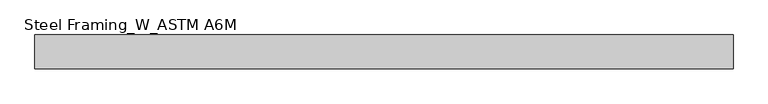
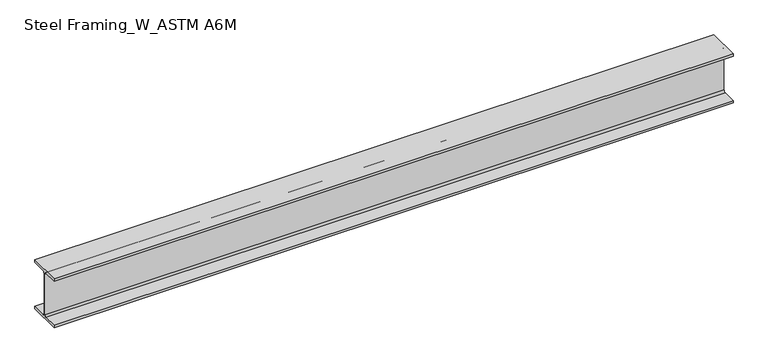
"""IFC4 building model written with IfcOpenShell, lengths in millimetres: beam geometry, Steel Framing_W_ASTM A6M : H_SB_AR_S02_W200x31.3_B6."""

from ifc_helpers import new_model, si_unit, point, frame, frame_2d, origin, place, context, project, spatial, polyline, circle_curve, trimmed, segment, composite_curve, outline, extrude, source, transform, mapped, element, save


def steel_framing_w_astm_a6m_88cf460a(model_context):
    return source(origin(), model_context, "Body", "SweptSolid", [
        extrude(outline(composite_curve([segment(polyline([(67.0, -94.8), (67.0, -105.0), (-67.0, -105.0), (-67.0, -94.8), (-10.775, -94.8)]), True, "CONTINUOUS"), segment(trimmed(circle_curve(frame_2d((-10.775, -87.2)), 7.6), [point((-10.775, -94.8))], [point((-3.175, -87.2))], True, "CARTESIAN"), True, "CONTINUOUS"), segment(polyline([(-3.175, -87.2), (-3.175, 87.2)]), True, "CONTINUOUS"), segment(trimmed(circle_curve(frame_2d((-10.775, 87.2)), 7.6), [point((-3.175, 87.2))], [point((-10.775, 94.8))], True, "CARTESIAN"), True, "CONTINUOUS"), segment(polyline([(-10.775, 94.8), (-67.0, 94.8), (-67.0, 105.0), (67.0, 105.0), (67.0, 94.8), (10.775, 94.8)]), True, "CONTINUOUS"), segment(trimmed(circle_curve(frame_2d((10.775, 87.2)), 7.6), [point((10.775, 94.8))], [point((3.175, 87.2))], True, "CARTESIAN"), True, "CONTINUOUS"), segment(polyline([(3.175, 87.2), (3.175, -87.2)]), True, "CONTINUOUS"), segment(trimmed(circle_curve(frame_2d((10.775, -87.2)), 7.6), [point((3.175, -87.2))], [point((10.775, -94.8))], True, "CARTESIAN"), True, "CONTINUOUS"), segment(polyline([(10.775, -94.8), (67.0, -94.8)]), True, "CONTINUOUS")], self_intersect=False)), frame((-1401.8, 0.0, 0.0), z_axis=(1.0, 0.0, 0.0), x_axis=(0.0, 1.0, 0.0)), (0.0, 0.0, 1.0), 2751.8),
    ])


if __name__ == "__main__":
    model = new_model("IFC4")
    model_context = context("Model", 3, world=origin())
    ifc_project = project(units=[si_unit("LENGTHUNIT", "METRE", prefix="MILLI")], contexts=[model_context])
    site = spatial("IfcSite", under=ifc_project)
    building = spatial("IfcBuilding", under=site)
    placement = place(None, origin())
    steel_framing_w_astm_a6m_shape = steel_framing_w_astm_a6m_88cf460a(model_context)
    element("IfcBeam", 1, ObjectType="Steel Framing_W_ASTM A6M : H_SB_AR_S02_W200x31.3_B6", at=placement, inside=building, context=model_context, shape_type="MappedRepresentation", body=[
        mapped(steel_framing_w_astm_a6m_shape, transform((0.0, 0.0, 0.0), x_axis=(1.0, 0.0, 0.0), y_axis=(0.0, 1.0, 0.0), z_axis=(0.0, 0.0, 1.0))),
    ])
    save(model, "model.ifc")

# Revit data of these elements
# Type "Steel Framing_W_ASTM A6M : H_SB_AR_S02_W200x31.3_B6"
#   Type Mark = "B6"
#   Section Name Key = "W8x21"
#   Width = 13.4 cm
#   Web Thickness = 0.635 cm
#   Web Fillet = 0.76 cm
#   Warping Constant = 40800.0 cm⁶
#   Torsional Moment of Inertia = 11.70 cm⁴
#   Section Area = 39.7 cm²
#   Plastic Modulus weak axis = 93.2 cm³
#   Plastic Modulus strong axis = 334.0 cm³
#   Perimeter = 0.93 m²/m
#   Nominal Weight = 31.30 kgf/m
#   Moment of Inertia weak axis = 407.00 cm⁴
#   Moment of Inertia strong axis = 3130.00 cm⁴
#   Height = 21.0 cm
#   Flange Thickness = 1.02 cm
#   Elastic Modulus weak axis = 60.8 cm³
#   Elastic Modulus strong axis = 298.0 cm³
#   Centroid Vertical = 10.5 cm
#   Centroid Horizontal = 6.7 cm
#   Length [instance default] = 1500 mm
#   Structural Material [instance default] = Steel, 45-345
#   Bolt Spacing = 0
#   Assembly Code = ""
# Element 1 (IfcBeam, "Steel Framing_W_ASTM A6M : H_SB_AR_S02_W200x31.3_B6")
#   Materials on its faces: "Steel, 45-345"
# Materials
#   "Steel, 45-345": class "Metal", colour RGB 189 187 185, transparency 0, Description = "Steel 345 MPa", Cost = 0
